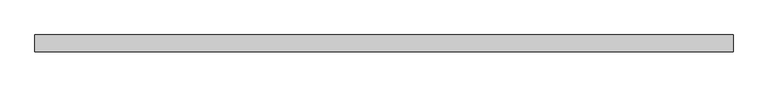
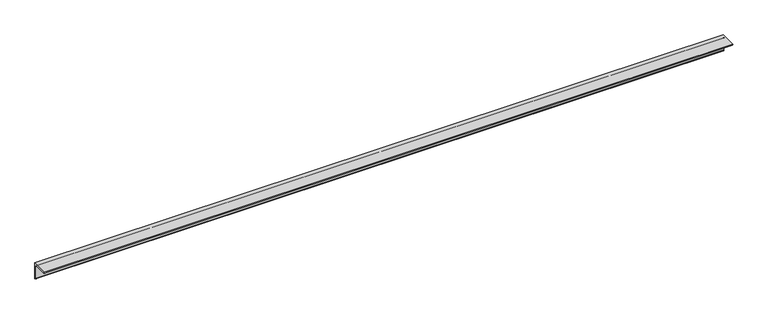
"""IFC4 building model written with IfcOpenShell, lengths in millimetres: member geometry, 0912_Steel Framing_L-KSD3502 : H_SB_AR_S03_L-130x130x12_HBR3."""

from ifc_helpers import new_model, si_unit, point, frame, frame_2d, origin, place, context, project, spatial, polyline, circle_curve, trimmed, segment, composite_curve, outline, extrude, source, transform, mapped, element, save


def member_6cc94826(model_context):
    return source(origin(), model_context, "Body", "SweptSolid", [
        extrude(outline(composite_curve([segment(polyline([(36.4, 36.4), (36.4, -93.6)]), True, "CONTINUOUS"), segment(trimmed(circle_curve(frame_2d((36.4, -81.6)), 12.0), [point((36.4, -93.6))], [point((24.4, -81.6))], False, "CARTESIAN"), True, "CONTINUOUS"), segment(polyline([(24.4, -81.6), (24.4, 12.4)]), True, "CONTINUOUS"), segment(trimmed(circle_curve(frame_2d((12.4, 12.4)), 12.0), [point((24.4, 12.4))], [point((12.4, 24.4))], True, "CARTESIAN"), True, "CONTINUOUS"), segment(polyline([(12.4, 24.4), (-81.6, 24.4)]), True, "CONTINUOUS"), segment(trimmed(circle_curve(frame_2d((-81.6, 36.4)), 12.0), [point((-81.6, 24.4))], [point((-93.6, 36.4))], False, "CARTESIAN"), True, "CONTINUOUS"), segment(polyline([(-93.6, 36.4), (36.4, 36.4)]), True, "CONTINUOUS")], self_intersect=False)), frame((-2682.0951934, 0.0, 0.0), z_axis=(1.0, 0.0, 0.0), x_axis=(0.0, 1.0, 0.0)), (0.0, 0.0, 1.0), 5417.5661112),
    ])


if __name__ == "__main__":
    model = new_model("IFC4")
    model_context = context("Model", 3, world=origin())
    ifc_project = project(units=[si_unit("LENGTHUNIT", "METRE", prefix="MILLI")], contexts=[model_context])
    site = spatial("IfcSite", under=ifc_project)
    building = spatial("IfcBuilding", under=site)
    placement = place(None, origin())
    member_shape = member_6cc94826(model_context)
    element("IfcMember", 1, ObjectType="0912_Steel Framing_L-KSD3502 : H_SB_AR_S03_L-130x130x12_HBR3", at=placement, inside=building, context=model_context, shape_type="MappedRepresentation", body=[
        mapped(member_shape, transform((0.0, 0.0, 0.0), x_axis=(1.0, 0.0, 0.0), y_axis=(0.0, 1.0, 0.0), z_axis=(0.0, 0.0, 1.0))),
    ])
    save(model, "model.ifc")

# Revit data of these elements
# Type "0912_Steel Framing_L-KSD3502 : H_SB_AR_S03_L-130x130x12_HBR3"
#   k = 25 mm
#   Perimeter = 0.52 m²/m
#   Nominal Weight = 23.40 kgf/m
#   Length [instance default] = 1000 mm
#   b = 130 mm
#   d = 130 mm
#   t = 12 mm
#   x = 36.4 mm
#   y = 36.4 mm
#   A = 2976.00 m²
#   Structural Material [instance default] = Steel, 45-345
# Element 1 (IfcMember, "0912_Steel Framing_L-KSD3502 : H_SB_AR_S03_L-130x130x12_HBR3")
#   Materials on its faces: "Steel, 45-345"
# Materials
#   "Steel, 45-345": class "Metal", colour RGB 189 187 185, transparency 0, Description = "Steel 345 MPa", Cost = 0
